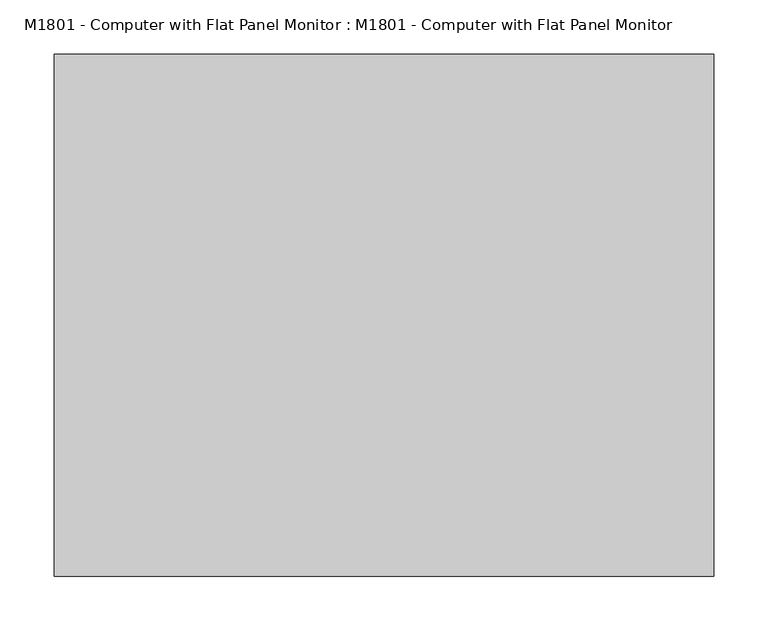
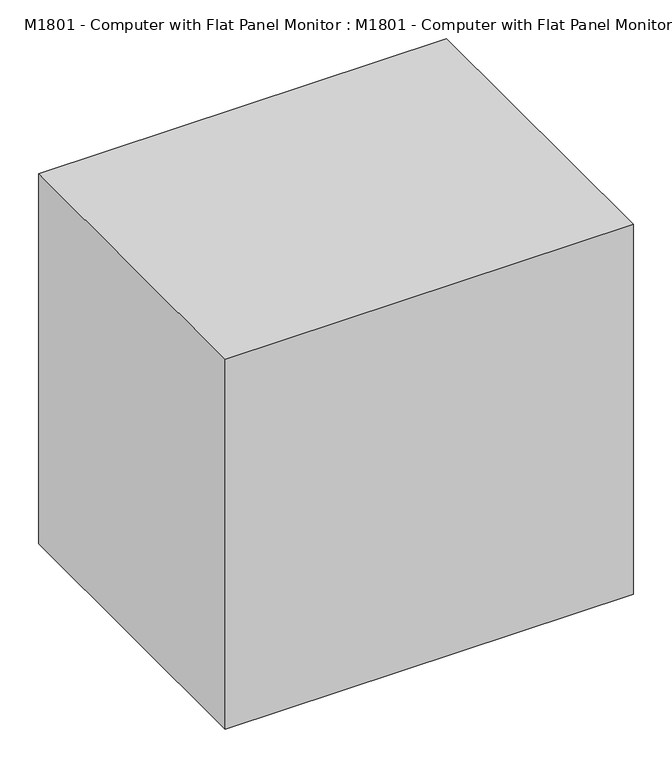
"""IFC4 building model written with IfcOpenShell, lengths in millimetres: proxy geometry, M1801 - Computer with Flat Panel Monitor : M1801 - Computer with Flat Panel Monitor."""

import ifcopenshell
import ifcopenshell.guid

model = None  # the IFC model being written
_history = None  # IfcOwnerHistory: only IFC2X3 demands one
_inside = {}  # id of a spatial element -> (the spatial element, [elements in it])
_under = {}  # id of a project, library or spatial element -> (it, [spatial elements below it])
_declared = {}  # id of a project -> (the project, [libraries it declares])
_typed = {}  # id of a type object -> (the type object, [elements of that type])
_made_of = {}  # id of a material, layer set ... -> (it, [elements and type objects made of it])


def new_model(schema):
    """Start an empty IFC model of exactly this schema.

    Asked for "IFC4X3", IfcOpenShell would pick the latest addendum, in which some entities
    have other attributes; the version numbers below select the first issue.
    IFC2X3 requires an IfcOwnerHistory on every rooted entity: one is made here for all.
    """
    global model, _history
    if schema == "IFC4X3":
        model = ifcopenshell.file(schema_version=(4, 3, 0, 0))
    else:
        model = ifcopenshell.file(schema=schema)
    _inside.clear()
    _under.clear()
    _declared.clear()
    _typed.clear()
    _made_of.clear()
    _history = None
    if model.schema == "IFC2X3":
        org = make("IfcOrganization", Name="unknown")
        user = make(
            "IfcPersonAndOrganization",
            ThePerson=make("IfcPerson", FamilyName="unknown"),
            TheOrganization=org,
        )
        app = make(
            "IfcApplication",
            ApplicationDeveloper=org,
            Version="unknown",
            ApplicationFullName="unknown",
            ApplicationIdentifier="unknown",
        )
        _history = make(
            "IfcOwnerHistory",
            OwningUser=user,
            OwningApplication=app,
            ChangeAction="ADDED",
            CreationDate=0,
        )
    return model


def make(cls, **values):
    """One entity of the class cls with the attributes given. An attribute that is None is left unset."""
    return model.create_entity(
        cls, **{name: value for name, value in values.items() if value is not None}
    )


def rooted(cls, **values):
    """An entity with a GlobalId (a new one), such as an element, a storey or a relation."""
    return make(cls, GlobalId=ifcopenshell.guid.new(), OwnerHistory=_history, **values)


def si_unit(unit_type, name, prefix=None):
    """IfcSIUnit, for example si_unit("LENGTHUNIT", "METRE", prefix="MILLI")."""
    return make("IfcSIUnit", UnitType=unit_type, Prefix=prefix, Name=name)


def assignment(units):
    """IfcUnitAssignment: the units of a project."""
    return None if units is None else make("IfcUnitAssignment", Units=units)


def point(xyz):
    """IfcCartesianPoint."""
    return None if xyz is None else make("IfcCartesianPoint", Coordinates=xyz)


def direction(xyz):
    """IfcDirection."""
    return None if xyz is None else make("IfcDirection", DirectionRatios=xyz)


def frame(location, z_axis=None, x_axis=None):
    """IfcAxis2Placement3D, a coordinate frame: its origin and axes. An axis left out is left unset."""
    return make(
        "IfcAxis2Placement3D",
        Location=point(location),
        Axis=direction(z_axis),
        RefDirection=direction(x_axis),
    )


def origin():
    """The frame at (0, 0, 0) with its axes left unset."""
    return frame((0.0, 0.0, 0.0))


def origin_with_axes():
    """The frame at (0, 0, 0) with the z axis (0, 0, 1) and the x axis (1, 0, 0) written out."""
    return frame((0.0, 0.0, 0.0), z_axis=(0.0, 0.0, 1.0), x_axis=(1.0, 0.0, 0.0))


def place(relative_to, where):
    """IfcLocalPlacement: puts the frame where relative to a parent placement (None: the world)."""
    return make(
        "IfcLocalPlacement", PlacementRelTo=relative_to, RelativePlacement=where
    )


def context(
    kind, dimensions, precision=None, world=None, true_north=None, identifier=None
):
    """IfcGeometricRepresentationContext, for example the 3D "Model" context."""
    return make(
        "IfcGeometricRepresentationContext",
        ContextIdentifier=identifier,
        ContextType=kind,
        CoordinateSpaceDimension=dimensions,
        Precision=precision,
        WorldCoordinateSystem=world,
        TrueNorth=true_north,
    )


def project(units=None, contexts=None):
    """IfcProject with its units and contexts."""
    return rooted(
        "IfcProject",
        Name="project",
        RepresentationContexts=contexts,
        UnitsInContext=assignment(units),
    )


def spatial(cls, under=None, at=None, **own):
    """A site, building, storey or space (cls), placed at a placement, below another one or the project."""
    s = rooted(cls, ObjectPlacement=at, **own)
    if under is not None:
        _under.setdefault(under.id(), (under, []))[1].append(s)
    return s


def polyline(points):
    """IfcPolyline through the points."""
    return make("IfcPolyline", Points=[point(p) for p in points])


def outline(outer, holes=None, kind="AREA"):
    """IfcArbitraryClosedProfileDef: a profile drawn as a closed curve; with holes, ...WithVoids."""
    if holes is None:
        return make("IfcArbitraryClosedProfileDef", ProfileType=kind, OuterCurve=outer)
    return make(
        "IfcArbitraryProfileDefWithVoids",
        ProfileType=kind,
        OuterCurve=outer,
        InnerCurves=holes,
    )


def extrude(swept, where, along, depth):
    """IfcExtrudedAreaSolid: the profile swept, set in the frame where, extruded along a direction by depth."""
    return make(
        "IfcExtrudedAreaSolid",
        SweptArea=swept,
        Position=where,
        ExtrudedDirection=direction(along),
        Depth=depth,
    )


def faces_of(points, faces, orient=None, outer=None):
    """IfcFace entities. A face is a list of loops; a loop is a list of indices into points, from 0.

    orient and outer hold one flag for each loop. By default every Orientation is true, the
    first loop of a face is its IfcFaceOuterBound and the others are IfcFaceBound.
    """
    made = []
    for i, loops in enumerate(faces):
        bounds = []
        for j, loop in enumerate(loops):
            is_outer = j == 0 if outer is None else outer[i][j]
            bounds.append(
                make(
                    "IfcFaceOuterBound" if is_outer else "IfcFaceBound",
                    Bound=make("IfcPolyLoop", Polygon=[points[k] for k in loop]),
                    Orientation=True if orient is None else orient[i][j],
                )
            )
        made.append(make("IfcFace", Bounds=bounds))
    return made


def faceted_brep(points, faces, orient=None, outer=None, voids=None):
    """IfcFacetedBrep: a solid bounded by flat faces; with voids (closed shells), ...WithVoids."""
    shared = [point(p) for p in points]
    hull = make("IfcClosedShell", CfsFaces=faces_of(shared, faces, orient, outer))
    if voids is None:
        return make("IfcFacetedBrep", Outer=hull)
    return make(
        "IfcFacetedBrepWithVoids",
        Outer=hull,
        Voids=[
            make(cls, CfsFaces=faces_of(shared, fs, o, b)) for cls, fs, o, b in voids
        ],
    )


def shape(context_of_items, identifier, shape_type, items):
    """IfcShapeRepresentation: the items that make up one representation, for example the "Body"."""
    return make(
        "IfcShapeRepresentation",
        ContextOfItems=context_of_items,
        RepresentationIdentifier=identifier,
        RepresentationType=shape_type,
        Items=items,
    )


def source(mapping_origin, context_of_items, identifier, shape_type, items):
    """IfcRepresentationMap: a shape defined once, which mapped items show again and again."""
    return make(
        "IfcRepresentationMap",
        MappingOrigin=mapping_origin,
        MappedRepresentation=shape(context_of_items, identifier, shape_type, items),
    )


def transform(
    local_origin,
    x_axis=None,
    y_axis=None,
    z_axis=None,
    scale=None,
    scale2=None,
    scale3=None,
    uniform=True,
):
    """IfcCartesianTransformationOperator3D, or its non-uniform kind. x_axis, y_axis, z_axis: its Axis1, 2, 3."""
    if uniform:
        return make(
            "IfcCartesianTransformationOperator3D",
            Axis1=direction(x_axis),
            Axis2=direction(y_axis),
            LocalOrigin=point(local_origin),
            Scale=scale,
            Axis3=direction(z_axis),
        )
    return make(
        "IfcCartesianTransformationOperator3DnonUniform",
        Axis1=direction(x_axis),
        Axis2=direction(y_axis),
        LocalOrigin=point(local_origin),
        Scale=scale,
        Axis3=direction(z_axis),
        Scale2=scale2,
        Scale3=scale3,
    )


def mapped(mapping_source, mapping_target):
    """IfcMappedItem: shows the shape of a source again, moved by a transform."""
    return make(
        "IfcMappedItem", MappingSource=mapping_source, MappingTarget=mapping_target
    )


def made_of(thing, what):
    """Note that an element or type object is made of a material, layer set ...; save() writes the relation."""
    if what is not None:
        _made_of.setdefault(what.id(), (what, []))[1].append(thing)
    return thing


def element(
    cls,
    number,
    at=None,
    inside=None,
    cuts=None,
    type_object=None,
    material=None,
    context=None,
    identifier="Body",
    shape_type=None,
    held_by="IfcProductDefinitionShape",
    body=None,
    shapes=None,
    **own,
):
    """One element of the class cls, such as IfcWall. Its Tag is "e" and its number.

    at: its placement. inside: the storey or other place that contains it. cuts: it is an
    opening in that element (IfcRelVoidsElement). A single representation is given by context,
    identifier, shape_type and body (its items); several are given by shapes. held_by: the class
    of the entity that holds the representations. save() writes the other relations.
    """
    e = rooted(cls, Tag="e%d" % number, ObjectPlacement=at, **own)
    if body is not None:
        shapes = [shape(context, identifier, shape_type, body)]
    if shapes is not None:
        e.Representation = make(held_by, Representations=shapes)
    if inside is not None:
        _inside.setdefault(inside.id(), (inside, []))[1].append(e)
    if cuts is not None:
        rooted(
            "IfcRelVoidsElement", RelatingBuildingElement=cuts, RelatedOpeningElement=e
        )
    if type_object is not None:
        _typed.setdefault(type_object.id(), (type_object, []))[1].append(e)
    return made_of(e, material)


def aggregate(whole, parts):
    """IfcRelAggregates: a whole, such as a stair, and the parts it consists of."""
    return rooted("IfcRelAggregates", RelatingObject=whole, RelatedObjects=parts)


def save(model, path):
    """Write the relations noted so far, then the file.

    IfcRelAggregates (storeys below a building ...), IfcRelContainedInSpatialStructure (elements
    in a storey), IfcRelDefinesByType, IfcRelAssociatesMaterial and IfcRelDeclares: one each for
    every whole, place, type object, material and project.
    """
    for whole, parts in _under.values():
        aggregate(whole, parts)
    for where, things in _inside.values():
        rooted(
            "IfcRelContainedInSpatialStructure",
            RelatedElements=things,
            RelatingStructure=where,
        )
    for kind, things in _typed.values():
        rooted("IfcRelDefinesByType", RelatedObjects=things, RelatingType=kind)
    for what, things in _made_of.values():
        rooted("IfcRelAssociatesMaterial", RelatedObjects=things, RelatingMaterial=what)
    for by, libraries in _declared.values():
        rooted("IfcRelDeclares", RelatingContext=by, RelatedDefinitions=libraries)
    model.write(path)


def m1801_computer_with_flat_panel_monitor_m1801_computer_with_1114ead5(model_context):
    return source(origin(), model_context, "Body", "SolidModel", [
        faceted_brep([(203.2, -133.2656905, 431.8), (203.2, -82.6343095, 431.8), (-203.2, -82.6343095, 431.8), (-203.2, -133.2656905, 431.8), (203.2, -133.2656905, 152.4), (-203.2, -133.2656905, 152.4), (-203.2, -82.6343095, 152.4), (203.2, -82.6343095, 152.4), (-190.5, -82.6343095, 419.1), (-190.5, -82.6343095, 165.1), (190.5, -82.6343095, 165.1), (190.5, -82.6343095, 419.1), (190.5, -87.4205119, 419.1), (-190.5, -87.4205119, 419.1), (190.5, -87.4205119, 165.1), (-190.5, -87.4205119, 165.1)], [[[0, 1, 2, 3]], [[4, 5, 6, 7]], [[3, 5, 4, 0]], [[2, 6, 5, 3]], [[1, 7, 6, 2], [8, 9, 10, 11]], [[0, 4, 7, 1]], [[12, 13, 8, 11]], [[14, 10, 9, 15]], [[12, 14, 15, 13]], [[13, 15, 9, 8]], [[11, 10, 14, 12]]]),
        faceted_brep([(109.1218395, -34.0676261, 25.4), (109.1218395, -215.9, 25.4), (109.1218395, -215.9, 0.0), (109.1218395, -34.0676261, 0.0), (-109.1218395, -215.9, 25.4), (-109.1218395, -34.0676261, 25.4), (-109.1218395, -34.0676261, 0.0), (-109.1218395, -215.9, 0.0), (36.9685686, -196.7656905, 31.75), (-36.9685686, -196.7656905, 31.75), (-36.9685686, -196.7656905, 25.4), (36.9685686, -196.7656905, 25.4), (36.9685686, -196.7656905, 292.1), (-36.9685686, -196.7656905, 292.1), (36.9685686, -133.2656905, 292.1), (-36.9685686, -133.2656905, 292.1), (36.9685686, -133.2656905, 241.3), (-36.9685686, -133.2656905, 241.3), (36.9685686, -171.3656905, 241.3), (-36.9685686, -171.3656905, 241.3), (36.9685686, -171.3656905, 25.4), (-36.9685686, -171.3656905, 25.4)], [[[0, 1, 2, 3]], [[4, 5, 6, 7]], [[8, 9, 10, 11]], [[12, 13, 9, 8]], [[14, 15, 13, 12]], [[16, 17, 15, 14]], [[18, 19, 17, 16]], [[20, 21, 19, 18]], [[0, 5, 4, 1], [11, 10, 21, 20]], [[3, 6, 5, 0]], [[2, 7, 6, 3]], [[1, 4, 7, 2]], [[20, 18, 16, 14, 12, 8, 11]], [[10, 9, 13, 15, 17, 19, 21]]]),
        extrude(outline(polyline([(171.45, 0.0), (19.05, 0.0), (19.05, 25.4), (171.45, 12.7), (171.45, 0.0)])), frame((-203.2, 0.0, 0.0), z_axis=(1.0, 0.0, 0.0), x_axis=(0.0, 1.0, 0.0)), (0.0, 0.0, 1.0), 406.4),
        extrude(outline(polyline([(304.8, -241.3), (-304.8, -241.3), (-304.8, 241.3), (304.8, 241.3), (304.8, -241.3)])), origin_with_axes(), (0.0, 0.0, 1.0), 584.2),
    ])


if __name__ == "__main__":
    model = new_model("IFC4")
    model_context = context("Model", 3, world=origin())
    ifc_project = project(units=[si_unit("LENGTHUNIT", "METRE", prefix="MILLI")], contexts=[model_context])
    site = spatial("IfcSite", under=ifc_project)
    building = spatial("IfcBuilding", under=site)
    placement = place(None, origin())
    m1801_computer_with_flat_panel_monitor_m1801_computer_with_shape = m1801_computer_with_flat_panel_monitor_m1801_computer_with_1114ead5(model_context)
    element("IfcBuildingElementProxy", 1, Name="M1801 - Computer with Flat Panel Monitor : M1801 - Computer with Flat Panel Monitor", ObjectType="M1801 - Computer with Flat Panel Monitor : M1801 - Computer with Flat Panel Monitor", at=placement, inside=building, context=model_context, shape_type="MappedRepresentation", body=[
        mapped(m1801_computer_with_flat_panel_monitor_m1801_computer_with_shape, transform((0.0, 0.0, 0.0), x_axis=(1.0, 0.0, 0.0), y_axis=(0.0, 1.0, 0.0), z_axis=(0.0, 0.0, 1.0))),
    ])
    save(model, "model.ifc")

# Revit data of these elements
# Project information
#   Room Abbreviation = "DNXS1"
#   Room Description = "Dental X-Ray, Extraoral/Panoramic/Cephlometric (DNXS1)"
#   Sheets - Total = "5"
#   Project Issue Date = "Issue Date"
#   Project Status = "Project Status"
#   Client Name = "Owner"
#   Project Address = "Enter address here"
#   Project Name = "Project Name"
#   Project Number = "Project Number"
#   Publication Date = "1-Feb-16"
# Type "M1801 - Computer with Flat Panel Monitor : M1801 - Computer with Flat Panel Monitor"
#   Watts2 = "0"
#   Watts1 = "600"
#   Unit_Issue = "EA"
#   UTIL_6_Misc = "-"
#   UTIL_5_NonMedGas = "-"
#   UTIL_4_MiscGas = "-"
#   UTIL_3_MedGas = "-"
#   UTIL_2_Elec = "A"
#   UTIL_1_WaterDrain = "-"
#   Nomenclature = "Computer, Microprocessing, w/Flat Panel Monitor"
#   NSN = "7025"
#   Location [instance default] = ""
#   JSN = "M1801"
#   Fund_Source_VA = "-"
#   Fund_Source_Navy = "-"
#   Fund_Source_Army = "-"
#   Fund_Source_AF = "-"
#   ELEC_Volts2 = "0"
#   ELEC_Volts1 = "120"
#   ELEC_Phase2 = "0"
#   ELEC_Phase1 = "1"
#   ELEC_HertzSwitch = "1"
#   ELEC_HertzDependent = "0"
#   ELEC_Hertz = "60"
#   ELEC_Amps2 = "0"
#   ELEC_Amps1 = "5"
#   DetailDescription = "Desk top microprocessing computer. The unit shall consist of a central processing mini tower, flat panel monitor, keyboard, mouse and speakers. The system shall have the following minimum characteristics: a 2.8 GHz Pentium processor; 512 MB memory; 80GB hard drive; 32/48x CD-ROMDVD combo; 1.44MB network interface card; video 32 MB NVIDIA; a 18 inch flat panel monitor. The computer is used throughout the facility to input, manipulate and retrieve information."
#   CAT_VA = "C"
#   CAT_Navy = "C"
#   CAT_IHS = "-"
#   CAT_Army = "C"
#   CAT_AF = "C"
#   BTUperhour = "0"
#   Weight_IP = 45
#   DIM_Width_IP = 2' - 0"
#   DIM_Height_IP = 1' - 11"
#   DIM_Depth_IP = 1' - 7"
#   Assembly Code = ""
# Element 1 (IfcBuildingElementProxy, "M1801 - Computer with Flat Panel Monitor : M1801 - Computer with Flat Panel Monitor")
#   Materials on its faces: "EquipSpace"
# Materials
#   "EquipSpace": class "Unassigned", colour RGB 221 217 195, transparency 0.5
